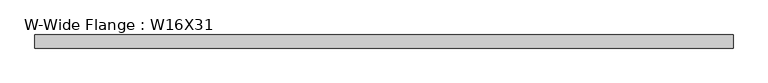
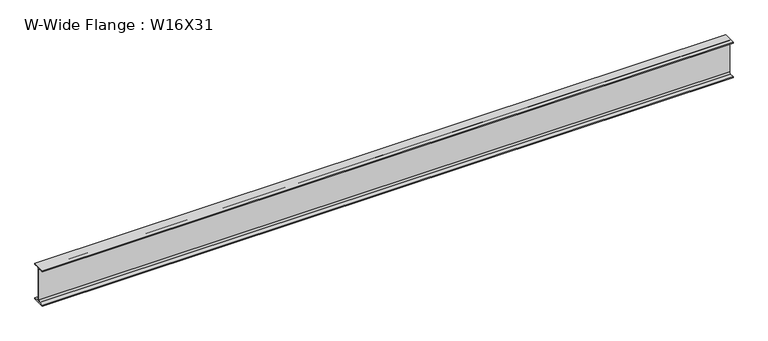
"""IFC4 building model written with IfcOpenShell, lengths in millimetres: beam geometry, W-Wide Flange : W16X31."""

from ifc_helpers import new_model, si_unit, point, frame, frame_2d, origin, place, context, project, spatial, polyline, circle_curve, trimmed, segment, composite_curve, outline, extrude, source, transform, mapped, element, save


def w_wide_flange_w16x31_e54a2e1a(model_context):
    return source(origin(), model_context, "Body", "SweptSolid", [
        extrude(outline(composite_curve([segment(polyline([(70.231, -190.754), (70.231, -201.93), (-70.231, -201.93), (-70.231, -190.754), (-20.8915, -190.754)]), True, "CONTINUOUS"), segment(trimmed(circle_curve(frame_2d((-20.8915, -173.355)), 17.399), [point((-20.8915, -190.754))], [point((-3.4925, -173.355))], True, "CARTESIAN"), True, "CONTINUOUS"), segment(polyline([(-3.4925, -173.355), (-3.4925, 173.355)]), True, "CONTINUOUS"), segment(trimmed(circle_curve(frame_2d((-20.8915, 173.355)), 17.399), [point((-3.4925, 173.355))], [point((-20.8915, 190.754))], True, "CARTESIAN"), True, "CONTINUOUS"), segment(polyline([(-20.8915, 190.754), (-70.231, 190.754), (-70.231, 201.93), (70.231, 201.93), (70.231, 190.754), (20.8915, 190.754)]), True, "CONTINUOUS"), segment(trimmed(circle_curve(frame_2d((20.8915, 173.355)), 17.399), [point((20.8915, 190.754))], [point((3.4925, 173.355))], True, "CARTESIAN"), True, "CONTINUOUS"), segment(polyline([(3.4925, 173.355), (3.4925, -173.355)]), True, "CONTINUOUS"), segment(trimmed(circle_curve(frame_2d((20.8915, -173.355)), 17.399), [point((3.4925, -173.355))], [point((20.8915, -190.754))], True, "CARTESIAN"), True, "CONTINUOUS"), segment(polyline([(20.8915, -190.754), (70.231, -190.754)]), True, "CONTINUOUS")], self_intersect=False)), frame((-3714.5535319, 0.0, 0.0), z_axis=(1.0, 0.0, 0.0), x_axis=(0.0, 1.0, 0.0)), (0.0, 0.0, 1.0), 7444.0959781),
    ])


if __name__ == "__main__":
    model = new_model("IFC4")
    model_context = context("Model", 3, world=origin())
    ifc_project = project(units=[si_unit("LENGTHUNIT", "METRE", prefix="MILLI")], contexts=[model_context])
    site = spatial("IfcSite", under=ifc_project)
    building = spatial("IfcBuilding", under=site)
    placement = place(None, origin())
    w_wide_flange_w16x31_shape = w_wide_flange_w16x31_e54a2e1a(model_context)
    element("IfcBeam", 1, ObjectType="W-Wide Flange : W16X31", at=placement, inside=building, context=model_context, shape_type="MappedRepresentation", body=[
        mapped(w_wide_flange_w16x31_shape, transform((0.0, 0.0, 0.0), x_axis=(1.0, 0.0, 0.0), y_axis=(0.0, 1.0, 0.0), z_axis=(0.0, 0.0, 1.0))),
    ])
    save(model, "model.ifc")

# Revit data of these elements
# Type "W-Wide Flange : W16X31"
#   Assembly Code = "B10"
#   W = 31
#   Start Extension Calculation [instance default] = 10' - 0"
#   Start Extension [instance default] = -0' - 0 1/2"
#   End Extension Calculation [instance default] = 10' - 0"
#   End Extension [instance default] = -0' - 0 1/2"
#   Length [instance default] = 5' - 0"
#   bf = 0' - 5.53"
#   d = 1' - 3.9"
#   k = 0' - 1 1/8"
#   k2 = 0' - 0.685"
#   tf = 0' - 0.44"
#   tw = 0' - 0.275"
#   A = 0.0634028 SF
#   Beam Material [instance default] = Metal - Steel - ASTM A992
# Element 1 (IfcBeam, "W-Wide Flange : W16X31")
#   Materials on its faces: "Metal - Steel - ASTM A992"
# Materials
#   "Metal - Steel - ASTM A992": class "Metal", colour RGB 128 0 0, transparency 0
